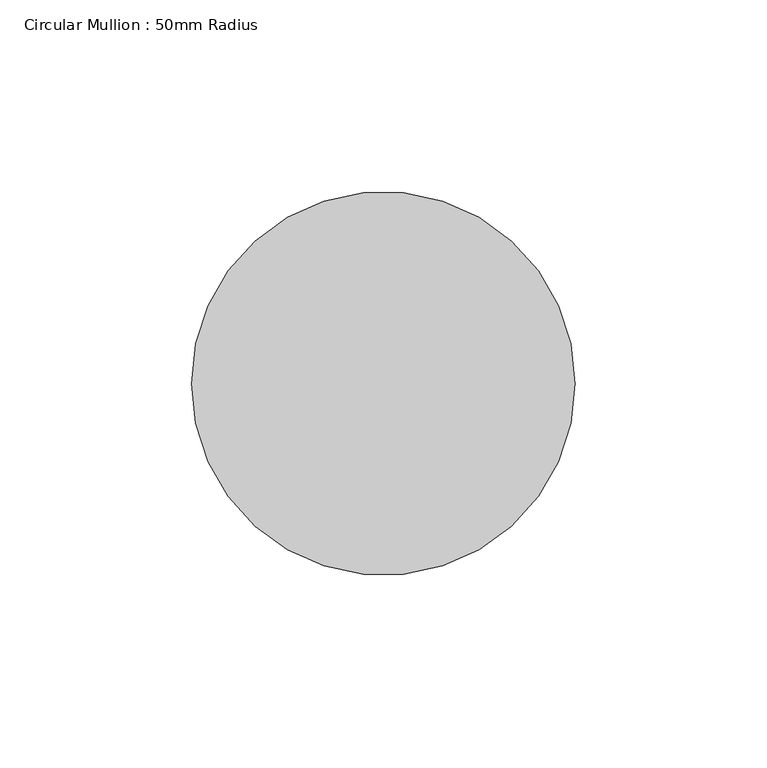
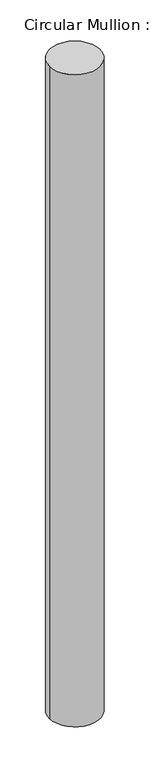
"""IFC4 building model written with IfcOpenShell, lengths in millimetres: member geometry, Circular Mullion : 50mm Radius."""

from ifc_helpers import new_model, si_unit, point, frame, origin, origin_2d, place, context, project, spatial, circle_curve, trimmed, segment, composite_curve, outline, extrude, source, transform, mapped, element, save


def circular_mullion_50mm_radius_5e2f0a11(model_context):
    return source(origin(), model_context, "Body", "SweptSolid", [
        extrude(outline(composite_curve([segment(trimmed(circle_curve(origin_2d(), 50.0), [point((50.0, 0.0))], [point((-50.0, 0.0))], False, "CARTESIAN"), True, "CONTINUOUS"), segment(trimmed(circle_curve(origin_2d(), 50.0), [point((-50.0, 0.0))], [point((50.0, 0.0))], False, "CARTESIAN"), True, "CONTINUOUS")], self_intersect=False)), frame((0.0, 0.0, -1356.304883), z_axis=(0.0, 0.0, 1.0), x_axis=(1.0, 0.0, 0.0)), (0.0, 0.0, 1.0), 1356.304883),
    ])


if __name__ == "__main__":
    model = new_model("IFC4")
    model_context = context("Model", 3, world=origin())
    ifc_project = project(units=[si_unit("LENGTHUNIT", "METRE", prefix="MILLI")], contexts=[model_context])
    site = spatial("IfcSite", under=ifc_project)
    building = spatial("IfcBuilding", under=site)
    placement = place(None, origin())
    circular_mullion_50mm_radius_shape = circular_mullion_50mm_radius_5e2f0a11(model_context)
    element("IfcMember", 1, ObjectType="Circular Mullion : 50mm Radius", at=placement, inside=building, context=model_context, shape_type="MappedRepresentation", body=[
        mapped(circular_mullion_50mm_radius_shape, transform((0.0, 0.0, 0.0), x_axis=(1.0, 0.0, 0.0), y_axis=(0.0, 1.0, 0.0), z_axis=(0.0, 0.0, 1.0))),
    ])
    save(model, "model.ifc")

# Revit data of these elements
# Type "Circular Mullion : 50mm Radius"
#   built-in parameter 1007350 = 0.164042 (stored number, unit not read)
# Element 1 (IfcMember, "Circular Mullion : 50mm Radius")
#   Materials on its faces: "Aluminium"
# Materials
#   "Aluminium": class "Metal", colour RGB 247 247 247, transparency 0, Description = "Aluminium 6061", Cost = 0
